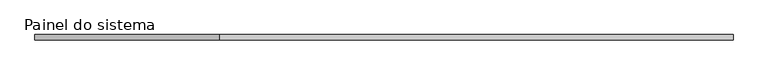
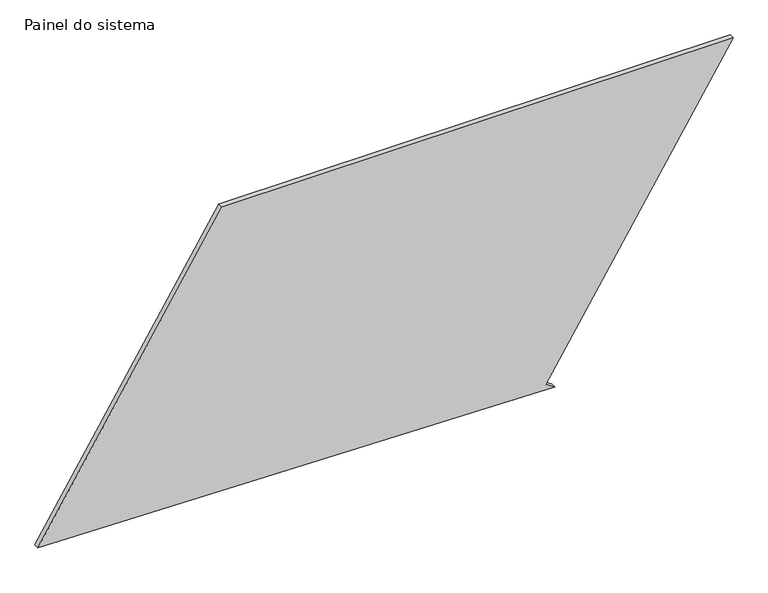
"""IFC4 building model written with IfcOpenShell, lengths in millimetres: plate geometry, Painel do sistema : Envidraçado."""

from ifc_helpers import new_model, si_unit, frame, origin, place, context, project, spatial, polyline, outline, extrude, source, transform, mapped, element, save


def painel_do_sistema_16fdf6be(model_context):
    return source(origin(), model_context, "Body", "SweptSolid", [
        extrude(outline(polyline([(0.0, 803.4919589), (26.4032514, 761.0317621), (1457.8390202, 1651.1491262), (1457.8390202, -776.8369034), (51.8201745, -1651.1491262), (0.0, 803.4919589)])), frame((0.0, 24.5, 0.0), z_axis=(0.0, 1.0, 0.0), x_axis=(0.0, 0.0, 1.0)), (0.0, 0.0, 1.0), 25.0),
    ])


if __name__ == "__main__":
    model = new_model("IFC4")
    model_context = context("Model", 3, world=origin())
    ifc_project = project(units=[si_unit("LENGTHUNIT", "METRE", prefix="MILLI")], contexts=[model_context])
    site = spatial("IfcSite", under=ifc_project)
    building = spatial("IfcBuilding", under=site)
    placement = place(None, origin())
    painel_do_sistema_shape = painel_do_sistema_16fdf6be(model_context)
    element("IfcPlate", 1, ObjectType="Painel do sistema : Envidraçado", at=placement, inside=building, context=model_context, shape_type="MappedRepresentation", body=[
        mapped(painel_do_sistema_shape, transform((0.0, 0.0, 0.0), x_axis=(1.0, 0.0, 0.0), y_axis=(0.0, 1.0, 0.0), z_axis=(0.0, 0.0, 1.0))),
    ])
    save(model, "model.ifc")

# Revit data of these elements
# Type "Painel do sistema : Envidraçado"
#   Construction Type Id = "GSP4R"
#   Analytic Construction = "Vidraça única Pilkington 1/8 pol"
#   Visual Light Transmittance = 0.9
#   Solar Heat Gain Coefficient = 0.86
#   Heat Transfer Coefficient (U) = 6.7069 W/(m²·K)
# Element 1 (IfcPlate, "Painel do sistema : Envidraçado")
#   Materials on its faces: "Vidro"
# Materials
#   "Vidro": class "Vidro", colour RGB 0 128 192, transparency 0.9, Description = "Vidro de sílica", Cost = 0
